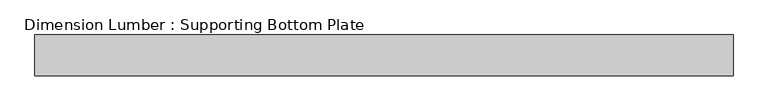
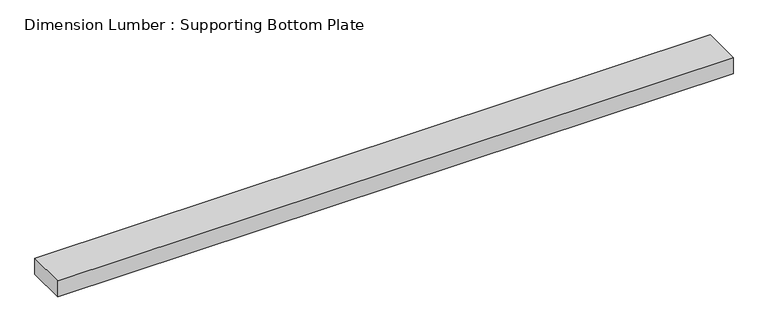
"""IFC4 building model written with IfcOpenShell, lengths in millimetres: beam geometry, Dimension Lumber : Supporting Bottom Plate."""

from ifc_helpers import new_model, si_unit, frame, origin, place, context, project, spatial, polyline, outline, extrude, source, transform, mapped, element, save


def dimension_lumber_supporting_bottom_plate_5d1fa65a(model_context):
    return source(origin(), model_context, "Body", "SweptSolid", [
        extrude(outline(polyline([(755.65, 44.45), (755.65, -44.45), (-755.65, -44.45), (-755.65, 44.45), (755.65, 44.45)])), frame((0.0, 0.0, -19.05), z_axis=(0.0, 0.0, 1.0), x_axis=(1.0, 0.0, 0.0)), (0.0, 0.0, 1.0), 38.1),
    ])


if __name__ == "__main__":
    model = new_model("IFC4")
    model_context = context("Model", 3, world=origin())
    ifc_project = project(units=[si_unit("LENGTHUNIT", "METRE", prefix="MILLI")], contexts=[model_context])
    site = spatial("IfcSite", under=ifc_project)
    building = spatial("IfcBuilding", under=site)
    placement = place(None, origin())
    dimension_lumber_supporting_bottom_plate_shape = dimension_lumber_supporting_bottom_plate_5d1fa65a(model_context)
    element("IfcBeam", 1, ObjectType="Dimension Lumber : Supporting Bottom Plate", at=placement, inside=building, context=model_context, shape_type="MappedRepresentation", body=[
        mapped(dimension_lumber_supporting_bottom_plate_shape, transform((0.0, 0.0, 0.0), x_axis=(1.0, 0.0, 0.0), y_axis=(0.0, 1.0, 0.0), z_axis=(0.0, 0.0, 1.0))),
    ])
    save(model, "model.ifc")

# Revit data of these elements
# Type "Dimension Lumber : Supporting Bottom Plate"
#   Assembly Code = "B10"
#   A = 0.0364583 SF
#   Length [instance default] = 5' - 0"
#   b = 0' - 3 1/2"
#   d = 0' - 1 1/2"
#   Structural Material [instance default] = Softwood, Lumber
# Element 1 (IfcBeam, "Dimension Lumber : Supporting Bottom Plate")
#   Structural Material = Douglas Fir #2
#   Materials on its faces: "Douglas Fir #2"
# Materials
#   "Softwood, Lumber": class "Wood", colour RGB 223 192 134, transparency 0, Description = "Pinus Echinata", Cost = 0
#   "Douglas Fir #2": class "Wood", colour RGB 223 192 134, transparency 0, Description = "Pinus Echinata", Cost = 0
